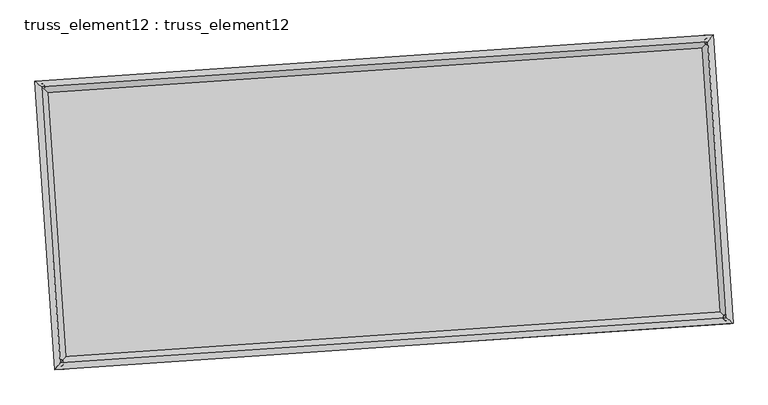
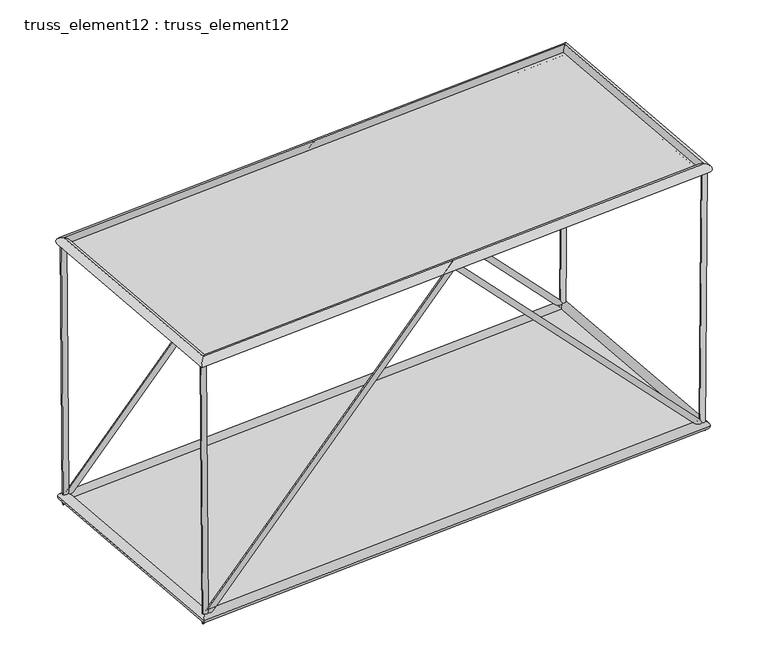
"""IFC4 building model written with IfcOpenShell, lengths in millimetres: plate geometry, truss_element12 : truss_element12."""

from ifc_helpers import new_model, si_unit, frame, origin, origin_with_axes, place, context, project, spatial, polyline, circle_curve, ellipse_curve, outline, extrude, source, transform, mapped, element, save
from ifc_brep_helpers import plane_surface, cylinder_surface, advanced_brep


def truss_element12_truss_element12_eab3e817(model_context):
    return source(origin(), model_context, "Body", "SolidModel", [
        advanced_brep(
        [(-3702.0882248, 2273.6910917, 5000.2328853), (-3801.1888293, 2260.330024, 4999.4898764), (-3665.8559791, 2276.1616308, 123.2430264), (-3763.1309037, 2262.9250493, -123.2430264), (1064.0216291, 2598.674005, 5071.9820203), (1064.4653189, 2592.1004843, 4927.7362277), (5793.3095347, 2921.1461695, 123.2387731), (5891.4514423, 2921.234319, -123.2387731), (5830.1270154, 2923.6566136, 5000.2343714), (5930.1239348, 2923.8712492, 4999.4793629)],
        [
            (0, 1, circle_curve(frame((-3751.638527, 2267.0105579, 4999.8613808), z_axis=(-0.00742901712052106, -0.0005065564371103783, 0.9999722761682941), x_axis=(-0.13361073627191278, 0.991033768581535, -0.0004905955135681844)), 50.0)),
            (1, 0, circle_curve(frame((-3751.638527, 2267.0105579, 4999.8613808), z_axis=(-0.00742901712052106, -0.0005065564371103783, 0.9999722761682941), x_axis=(-0.13361073627191278, 0.991033768581535, -0.0004905955135681844)), 50.0)),
            (0, 2),
            (2, 3, ellipse_curve(frame((-3714.4934414, 2269.54334, 0.0), z_axis=(-0.9271592320010837, -0.06321946356795351, 0.36929535326258994), x_axis=(0.3684398421976921, 0.025122512268499236, 0.9293120800133068)), 132.9062538, 50.0)),
            (3, 1),
            (3, 2, ellipse_curve(frame((-3714.4934414, 2269.54334, 0.0), z_axis=(-0.9271592320010837, -0.06321946356795351, 0.36929535326258994), x_axis=(0.3684398421976921, 0.025122512268499236, 0.9293120800133068)), 132.9062538, 50.0)),
            (2, 4),
            (4, 5, ellipse_curve(frame((1064.243474, 2595.3872446, 4999.859124), z_axis=(-0.9976833955843889, -0.0680282381952549, 3.1356873965195084e-05), x_axis=(-3.128423250774107e-05, -2.1331528923241756e-06, -0.9999999995083731)), 72.2799434, 50.0)),
            (5, 3),
            (5, 4, ellipse_curve(frame((1064.243474, 2595.3872446, 4999.859124), z_axis=(-0.9976833955843889, -0.0680282381952549, 3.1356873965195084e-05), x_axis=(-3.128423250774107e-05, -2.1331528923241756e-06, -0.9999999995083731)), 72.2799434, 50.0)),
            (4, 6),
            (6, 7, ellipse_curve(frame((5842.3804885, 2921.1902443, 0.0), z_axis=(-0.9271929359308114, -0.06322176171080063, -0.369210330849754), x_axis=(-0.3683550167481115, -0.025116728343544018, 0.929345862202988)), 132.8968359, 50.0)),
            (7, 5),
            (7, 6, ellipse_curve(frame((5842.3804885, 2921.1902443, 0.0), z_axis=(-0.9271929359308114, -0.06322176171080063, -0.369210330849754), x_axis=(-0.3683550167481115, -0.025116728343544018, 0.929345862202988)), 132.8968359, 50.0)),
            (8, 9, circle_curve(frame((5880.1254751, 2923.7639314, 4999.8568672), z_axis=(0.007548997314579444, 0.0005147374304556931, 0.999971373432721), x_axis=(-0.002150181299370391, 0.9999975640967588, -0.0004985187346304086)), 50.0)),
            (9, 8, circle_curve(frame((5880.1254751, 2923.7639314, 4999.8568672), z_axis=(0.007548997314579444, 0.0005147374304556931, 0.999971373432721), x_axis=(-0.002150181299370391, 0.9999975640967588, -0.0004985187346304086)), 50.0)),
            (6, 8),
            (9, 7),
        ],
        [
            plane_surface(frame((-3751.638527, 2317.0105514, 4999.8867094), z_axis=(-0.007429017120522367, -0.0005065564371127931, 0.9999722761682941), x_axis=(0.9999724044715549, -3.7633202945031043e-06, 0.007429016167328942))),
            cylinder_surface(frame((-3751.638527, 2267.0105579, 4999.8613808), z_axis=(-0.00742901712052106, -0.0005065564371103783, 0.9999722761682941), x_axis=(-0.13361073627191278, 0.991033768581535, -0.0004905955135681844)), 50.0),
            cylinder_surface(frame((-3714.4934414, 2269.54334, 0.0), z_axis=(-0.6901748995971244, -0.04706040280311354, -0.7221107438988209), x_axis=(-0.020414552183437053, 0.998752186075548, -0.045577591736113365)), 50.0),
            cylinder_surface(frame((1064.243474, 2595.3872446, 4999.859124), z_axis=(-0.6901297168790954, -0.047057321965326554, 0.7221541264368925), x_axis=(-0.11534915767572501, 0.9922789562072498, -0.04557460797145166)), 50.0),
            plane_surface(frame((5880.1254751, 2873.763938, 4999.8826048), z_axis=(0.007548997314579199, 0.0005147374304560268, 0.999971373432721), x_axis=(0.9999715059138159, -3.885862204455747e-06, -0.007548996314451271))),
            cylinder_surface(frame((5842.3804885, 2921.1902443, 0.0), z_axis=(-0.007548997314579444, -0.0005147374304556931, -0.999971373432721), x_axis=(-0.002150181299370391, 0.9999975640967588, -0.0004985187346304086)), 50.0),
        ],
        [
            (0, [[1, 2]]),
            (1, [[-1, 3, 4, 5]]),
            (1, [[-2, -5, 6, -3]]),
            (2, [[-4, 7, 8, 9]]),
            (2, [[-6, -9, 10, -7]]),
            (3, [[-8, 11, 12, 13]]),
            (3, [[-10, -13, 14, -11]]),
            (4, [[15, 16]]),
            (5, [[-12, 17, -16, 18]]),
            (5, [[-14, -18, -15, -17]]),
        ],
    ),
        advanced_brep(
        [(-3429.9752719, -1717.0424926, 5000.2328853), (-3529.0758763, -1730.4035603, 4999.4898764), (-3393.7430262, -1714.5719535, 123.2430264), (-3491.0179508, -1727.808535, -123.2430264), (1336.1345821, -1392.0595793, 5071.9820203), (1336.5782718, -1398.6331, 4927.7362277), (6065.4224876, -1069.5874148, 123.2387731), (6163.5643952, -1069.4992653, -123.2387731), (6102.2399683, -1067.0769707, 5000.2343714), (6202.2368877, -1066.8623351, 4999.4793629)],
        [
            (0, 1, circle_curve(frame((-3479.5255741, -1723.7230264, 4999.8613808), z_axis=(-0.007429017120521156, -0.0005065564371104173, 0.9999722761682941), x_axis=(-0.1336107362719125, 0.9910337685815351, -0.0004905955135681566)), 50.0)),
            (1, 0, circle_curve(frame((-3479.5255741, -1723.7230264, 4999.8613808), z_axis=(-0.007429017120521156, -0.0005065564371104173, 0.9999722761682941), x_axis=(-0.1336107362719125, 0.9910337685815351, -0.0004905955135681566)), 50.0)),
            (0, 2),
            (2, 3, ellipse_curve(frame((-3442.3804885, -1721.1902443, 0.0), z_axis=(-0.9271592320010837, -0.06321946356795342, 0.3692953532625894), x_axis=(0.3684398421976915, 0.025122512268499122, 0.929312080013307)), 132.9062538, 50.0)),
            (3, 1),
            (3, 2, ellipse_curve(frame((-3442.3804885, -1721.1902443, 0.0), z_axis=(-0.9271592320010837, -0.06321946356795342, 0.3692953532625894), x_axis=(0.3684398421976915, 0.025122512268499122, 0.929312080013307)), 132.9062538, 50.0)),
            (2, 4),
            (4, 5, ellipse_curve(frame((1336.3564269, -1395.3463397, 4999.859124), z_axis=(-0.9976833955843889, -0.068028238195255, 3.135687396423212e-05), x_axis=(-3.128423250681861e-05, -2.1331528920455174e-06, -0.9999999995083731)), 72.2799434, 50.0)),
            (5, 3),
            (5, 4, ellipse_curve(frame((1336.3564269, -1395.3463397, 4999.859124), z_axis=(-0.9976833955843889, -0.068028238195255, 3.135687396423212e-05), x_axis=(-3.128423250681861e-05, -2.1331528920455174e-06, -0.9999999995083731)), 72.2799434, 50.0)),
            (4, 6),
            (6, 7, ellipse_curve(frame((6114.4934414, -1069.54334, 0.0), z_axis=(-0.9271929359308113, -0.06322176171080102, -0.36921033084975446), x_axis=(-0.36835501674811183, -0.025116728343544108, 0.9293458622029878)), 132.8968359, 50.0)),
            (7, 5),
            (7, 6, ellipse_curve(frame((6114.4934414, -1069.54334, 0.0), z_axis=(-0.9271929359308113, -0.06322176171080102, -0.36921033084975446), x_axis=(-0.36835501674811183, -0.025116728343544108, 0.9293458622029878)), 132.8968359, 50.0)),
            (8, 9, circle_curve(frame((6152.238428, -1066.9696529, 4999.8568672), z_axis=(0.0075489973145789376, 0.0005147374304557482, 0.9999713734327209), x_axis=(-0.002150181299370522, 0.9999975640967588, -0.0004985187346304639)), 50.0)),
            (9, 8, circle_curve(frame((6152.238428, -1066.9696529, 4999.8568672), z_axis=(0.0075489973145789376, 0.0005147374304557482, 0.9999713734327209), x_axis=(-0.002150181299370522, 0.9999975640967588, -0.0004985187346304639)), 50.0)),
            (6, 8),
            (9, 7),
        ],
        [
            plane_surface(frame((-3479.5255741, -1673.7230329, 4999.8867094), z_axis=(-0.007429017120522367, -0.000506556437112789, 0.9999722761682941), x_axis=(0.9999724044715549, -3.7633202945031043e-06, 0.007429016167328942))),
            cylinder_surface(frame((-3479.5255741, -1723.7230264, 4999.8613808), z_axis=(-0.007429017120521158, -0.0005065564371104174, 0.9999722761682943), x_axis=(-0.1336107362719125, 0.9910337685815351, -0.0004905955135681566)), 50.0),
            cylinder_surface(frame((-3442.3804885, -1721.1902443, 0.0), z_axis=(-0.6901748995971234, -0.04706040280311338, -0.7221107438988217), x_axis=(-0.020414552183436876, 0.998752186075548, -0.0455775917361133)), 50.0),
            cylinder_surface(frame((1336.3564269, -1395.3463397, 4999.859124), z_axis=(-0.6901297168790961, -0.04705732196532681, 0.7221541264368919), x_axis=(-0.11534915767572519, 0.9922789562072498, -0.04557460797145163)), 50.0),
            plane_surface(frame((6152.238428, -1116.9696463, 4999.8826048), z_axis=(0.007548997314579199, 0.0005147374304560219, 0.999971373432721), x_axis=(0.9999715059138159, -3.885862204455747e-06, -0.007548996314451271))),
            cylinder_surface(frame((6114.4934414, -1069.54334, 0.0), z_axis=(-0.007548997314578939, -0.0005147374304557483, -0.9999713734327211), x_axis=(-0.002150181299370522, 0.9999975640967588, -0.0004985187346304639)), 50.0),
        ],
        [
            (0, [[1, 2]]),
            (1, [[-1, 3, 4, 5]]),
            (1, [[-2, -5, 6, -3]]),
            (2, [[-4, 7, 8, 9]]),
            (2, [[-6, -9, 10, -7]]),
            (3, [[-8, 11, 12, 13]]),
            (3, [[-10, -13, 14, -11]]),
            (4, [[15, 16]]),
            (5, [[-12, 17, -16, 18]]),
            (5, [[-14, -18, -15, -17]]),
        ],
    ),
        advanced_brep(
        [(-3479.5267648, -1723.7243462, 4909.8613809), (-3479.5243834, -1723.7217067, 5089.8613808), (-3751.6371682, 2267.009412, 5089.8613808), (-3751.6398859, 2267.0117037, 4909.8613809), (5880.1243683, 2923.7626174, 5089.8568672), (5880.1265818, 2923.7652454, 4909.8568672), (6152.2371531, -1066.9685013, 5089.8568672), (6152.2397029, -1066.9708045, 4909.8568672)],
        [
            (0, 1, ellipse_curve(frame((-3479.5255741, -1723.7230264, 4999.8613808), z_axis=(-0.7535719234053809, 0.6573654662780861, 3.30599714592259e-07), x_axis=(-0.6573654662780039, -0.7535719234054525, 3.305997145922409e-07)), 127.2792206, 90.0)),
            (1, 2),
            (2, 3, ellipse_curve(frame((-3751.638527, 2267.0105579, 4999.8613808), z_axis=(-0.6573654662780037, -0.7535719234054528, 3.3059971459222477e-07), x_axis=(0.7535719234053809, -0.657365466278086, -3.305997145922429e-07)), 127.2792206, 90.0)),
            (3, 0),
            (1, 0, ellipse_curve(frame((-3479.5255741, -1723.7230264, 4999.8613808), z_axis=(-0.7535719234053809, 0.6573654662780861, 3.30599714592259e-07), x_axis=(-0.6573654662780039, -0.7535719234054525, 3.305997145922409e-07)), 127.2792206, 90.0)),
            (3, 2, ellipse_curve(frame((-3751.638527, 2267.0105579, 4999.8613808), z_axis=(-0.6573654662780037, -0.7535719234054528, 3.3059971459222477e-07), x_axis=(0.7535719234053809, -0.657365466278086, -3.305997145922429e-07)), 127.2792206, 90.0)),
            (2, 4),
            (4, 5, ellipse_curve(frame((5880.1254751, 2923.7639314, 4999.8568672), z_axis=(-0.7535719234053808, 0.6573654662780862, 3.3059971459222667e-07), x_axis=(-0.6573654662780037, -0.7535719234054528, 3.3059971459224097e-07)), 127.2792206, 90.0)),
            (5, 3),
            (5, 4, ellipse_curve(frame((5880.1254751, 2923.7639314, 4999.8568672), z_axis=(-0.7535719234053808, 0.6573654662780862, 3.3059971459222667e-07), x_axis=(-0.6573654662780037, -0.7535719234054528, 3.3059971459224097e-07)), 127.2792206, 90.0)),
            (4, 6),
            (6, 7, ellipse_curve(frame((6152.238428, -1066.9696529, 4999.8568672), z_axis=(0.6573654662780037, 0.7535719234054526, -3.3059971459225706e-07), x_axis=(-0.7535719234053807, 0.6573654662780862, 3.3059971459224277e-07)), 127.2792206, 90.0)),
            (7, 5),
            (7, 6, ellipse_curve(frame((6152.238428, -1066.9696529, 4999.8568672), z_axis=(0.6573654662780037, 0.7535719234054526, -3.3059971459225706e-07), x_axis=(-0.7535719234053807, 0.6573654662780862, 3.3059971459224277e-07)), 127.2792206, 90.0)),
            (6, 1),
            (0, 7),
        ],
        [
            cylinder_surface(frame((-3479.5255741, -1723.7230264, 4999.8613808), z_axis=(0.06802823822870098, -0.9976833960748767, 0.0), x_axis=(-0.9976833959743321, -0.06802823822184523, 1.4197044503846432e-05)), 90.0),
            cylinder_surface(frame((-3751.638527, 2267.0105579, 4999.8613808), z_axis=(-0.9976833960747676, -0.06802823822869408, 4.6753860009301154e-07), x_axis=(-0.06802823821588568, 0.997683395981282, 1.3729505903797475e-05)), 90.0),
            cylinder_surface(frame((5880.1254751, 2923.7639314, 4999.8568672), z_axis=(-0.06802823822870059, 0.9976833960748767, 0.0), x_axis=(0.9976833959871405, 0.0680282382227182, 1.3261967303748516e-05)), 90.0),
            cylinder_surface(frame((6152.238428, -1066.9696529, 4999.8568672), z_axis=(0.9976833960747675, 0.06802823822869422, -4.6753860009303425e-07), x_axis=(0.06802823822869422, -0.9976833959804086, 1.3729505903797473e-05)), 90.0),
        ],
        [
            (0, [[1, 2, 3, 4]]),
            (0, [[5, -4, 6, -2]]),
            (1, [[-3, 7, 8, 9]]),
            (1, [[-6, -9, 10, -7]]),
            (2, [[-8, 11, 12, 13]]),
            (2, [[-10, -13, 14, -11]]),
            (3, [[-12, 15, -1, 16]]),
            (3, [[-14, -16, -5, -15]]),
        ],
    ),
        advanced_brep(
        [(-3358.7115243, -1625.2761972, 0.0), (-3526.0494527, -1817.1042913, 0.0), (-3810.4074885, 2353.2123043, 0.0), (-3618.5793943, 2185.8743758, 0.0), (5926.0494527, 3017.1042913, 0.0), (5758.7115243, 2825.2761972, 0.0), (6210.4074885, -1153.2123043, 0.0), (6018.5793943, -985.8743758, 0.0)],
        [
            (0, 1, ellipse_curve(frame((-3442.3804885, -1721.1902443, 0.0), z_axis=(-0.7535719234054562, 0.6573654662780827, 0.0), x_axis=(-0.6573654662780827, -0.7535719234054564, 0.0)), 127.2792206, 90.0)),
            (1, 2),
            (2, 3, ellipse_curve(frame((-3714.4934414, 2269.54334, 0.0), z_axis=(-0.6573654662780826, -0.7535719234054563, 0.0), x_axis=(0.7535719234054563, -0.6573654662780828, 0.0)), 127.2792206, 90.0)),
            (3, 0),
            (1, 0, ellipse_curve(frame((-3442.3804885, -1721.1902443, 0.0), z_axis=(-0.7535719234054562, 0.6573654662780827, 0.0), x_axis=(-0.6573654662780827, -0.7535719234054564, 0.0)), 127.2792206, 90.0)),
            (3, 2, ellipse_curve(frame((-3714.4934414, 2269.54334, 0.0), z_axis=(-0.6573654662780826, -0.7535719234054563, 0.0), x_axis=(0.7535719234054563, -0.6573654662780828, 0.0)), 127.2792206, 90.0)),
            (2, 4),
            (4, 5, ellipse_curve(frame((5842.3804885, 2921.1902443, 0.0), z_axis=(-0.7535719234054563, 0.6573654662780827, 0.0), x_axis=(-0.6573654662780828, -0.7535719234054563, 0.0)), 127.2792206, 90.0)),
            (5, 3),
            (5, 4, ellipse_curve(frame((5842.3804885, 2921.1902443, 0.0), z_axis=(-0.7535719234054563, 0.6573654662780827, 0.0), x_axis=(-0.6573654662780828, -0.7535719234054563, 0.0)), 127.2792206, 90.0)),
            (4, 6),
            (6, 7, ellipse_curve(frame((6114.4934414, -1069.54334, 0.0), z_axis=(0.6573654662780828, 0.7535719234054562, 0.0), x_axis=(-0.7535719234054563, 0.6573654662780828, 0.0)), 127.2792206, 90.0)),
            (7, 5),
            (7, 6, ellipse_curve(frame((6114.4934414, -1069.54334, 0.0), z_axis=(0.6573654662780828, 0.7535719234054562, 0.0), x_axis=(-0.7535719234054563, 0.6573654662780828, 0.0)), 127.2792206, 90.0)),
            (6, 1),
            (0, 7),
        ],
        [
            cylinder_surface(frame((-3442.3804885, -1721.1902443, 0.0), z_axis=(0.06802823822869855, -0.9976833960748768, 0.0), x_axis=(-0.9976833960748768, -0.06802823822869855, 0.0)), 90.0),
            cylinder_surface(frame((-3714.4934414, 2269.54334, 0.0), z_axis=(-0.9976833960748768, -0.0680282382286992, 0.0), x_axis=(-0.0680282382286992, 0.9976833960748768, 0.0)), 90.0),
            cylinder_surface(frame((5842.3804885, 2921.1902443, 0.0), z_axis=(-0.0680282382286982, 0.9976833960748769, 0.0), x_axis=(0.9976833960748769, 0.0680282382286982, 0.0)), 90.0),
            cylinder_surface(frame((6114.4934414, -1069.54334, 0.0), z_axis=(0.9976833960748768, 0.06802823822869884, 0.0), x_axis=(0.06802823822869884, -0.9976833960748768, 0.0)), 90.0),
        ],
        [
            (0, [[1, 2, 3, 4]]),
            (0, [[5, -4, 6, -2]]),
            (1, [[-3, 7, 8, 9]]),
            (1, [[-6, -9, 10, -7]]),
            (2, [[-8, 11, 12, 13]]),
            (2, [[-10, -13, 14, -11]]),
            (3, [[-12, 15, -1, 16]]),
            (3, [[-14, -16, -5, -15]]),
        ],
    ),
        extrude(outline(polyline([(-3442.3804885, -1721.1902443), (-3714.4934414, 2269.54334), (5842.3804885, 2921.1902443), (6114.4934414, -1069.54334), (-3442.3804885, -1721.1902443)])), origin_with_axes(), (0.0, 0.0, 1.0), 20.0),
        extrude(outline(polyline([(-2000.0, 4827.0643974), (2000.0, 4827.0643974), (2000.0, -4827.0643974), (-2000.0, -4827.0643974), (-2000.0, 4827.0643974)])), frame((1200.2999505, 600.0204525, 4999.859124), z_axis=(4.664554983369009e-07, 3.180582726824052e-08, 0.9999999999998908), x_axis=(-0.06802823822869884, 0.9976833960748768, 0.0)), (0.0, 0.0, 1.0), 20.0),
    ])


if __name__ == "__main__":
    model = new_model("IFC4")
    model_context = context("Model", 3, world=origin())
    ifc_project = project(units=[si_unit("LENGTHUNIT", "METRE", prefix="MILLI")], contexts=[model_context])
    site = spatial("IfcSite", under=ifc_project)
    building = spatial("IfcBuilding", under=site)
    placement = place(None, origin())
    truss_element12_truss_element12_shape = truss_element12_truss_element12_eab3e817(model_context)
    element("IfcPlate", 1, ObjectType="truss_element12 : truss_element12", at=placement, inside=building, context=model_context, shape_type="MappedRepresentation", body=[
        mapped(truss_element12_truss_element12_shape, transform((0.0, 0.0, 0.0), x_axis=(1.0, 0.0, 0.0), y_axis=(0.0, 1.0, 0.0), z_axis=(0.0, 0.0, 1.0))),
    ])
    save(model, "model.ifc")

# Revit data of these elements
# Type "truss_element12 : truss_element12"
#   steellbar1 = 90 mm
#   steelbar2 = 50 mm
#   offset1 = 5000 mm
#   M = Default Roof
# Element 1 (IfcPlate, "truss_element12 : truss_element12")
#   Materials on its faces: "Default Roof"
# Materials
#   "Default Roof": class "Miscellaneous", colour RGB 0 127 0, transparency 0, Comments = "Rendering appearance not upgraded Rendering appearance not upgraded ", Cost = 0
